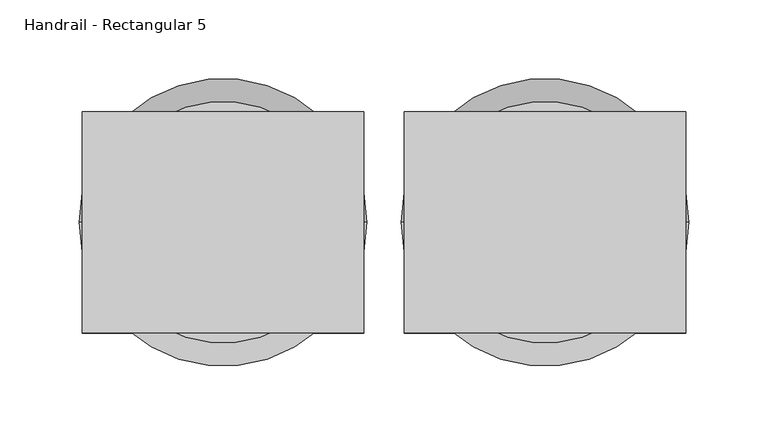
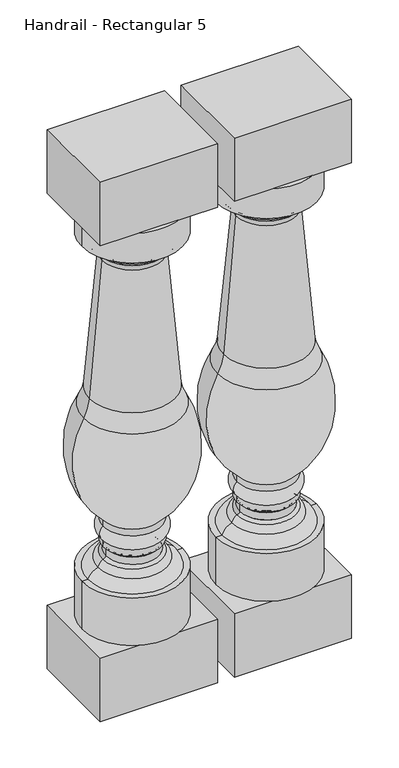
"""IFC4 building model written with IfcOpenShell, lengths in millimetres: railing geometry, Handrail - Rectangular 5."""

from ifc_helpers import new_model, si_unit, point, frame, origin, place, context, project, spatial, polyline, circle_curve, ellipse_curve, trimmed, outline, extrude, source, transform, mapped, element, save
from ifc_brep_helpers import plane_surface, cylinder_surface, revolved_surface, advanced_brep


def handrail_rectangular_5_6e42911b(model_context):
    return source(origin(), model_context, "Body", "SolidModel", [
        advanced_brep(
        [(16494.6521895, -1665.6164768, 873.125), (16647.0521895, -1665.6164768, 873.125), (16570.8521895, -1665.6164768, 873.125), (16494.6521895, -1665.6164768, 825.4490755), (16647.0521895, -1665.6164768, 825.4490755), (16504.6954208, -1665.6164768, 825.4490755), (16637.0089583, -1665.6164768, 825.4490755), (16516.1787107, -1665.6164768, 813.9657856), (16625.5256684, -1665.6164768, 813.9657856), (16516.1787107, -1665.6164768, 808.3461292), (16625.5256684, -1665.6164768, 808.3461292), (16521.8808978, -1665.6164768, 802.2016975), (16619.8234813, -1665.6164768, 802.2016975), (16525.2226936, -1665.6164768, 792.8428746), (16616.4816855, -1665.6164768, 792.8428746), (16506.4551876, -1665.6164768, 577.4758218), (16635.2491915, -1665.6164768, 577.4758218), (16497.437965, -1665.6164768, 549.5125844), (16644.2664141, -1665.6164768, 549.5125844), (16526.7087972, -1665.6164768, 376.7693301), (16614.9955818, -1665.6164768, 376.7693301), (16526.7087972, -1665.6164768, 366.4437154), (16614.9955818, -1665.6164768, 366.4437154), (16526.7087972, -1665.6164768, 343.8682651), (16614.9955818, -1665.6164768, 343.8682651), (16526.7087972, -1665.6164768, 333.5426504), (16614.9955818, -1665.6164768, 333.5426504), (16531.0192375, -1665.6164768, 329.2322102), (16610.6851416, -1665.6164768, 329.2322102), (16531.0192375, -1665.6164768, 317.4353211), (16610.6851416, -1665.6164768, 317.4353211), (16526.5214444, -1665.6164768, 313.1289544), (16615.1829347, -1665.6164768, 313.1289544), (16519.0009874, -1665.6164768, 303.0807869), (16622.7033917, -1665.6164768, 303.0807869), (16503.8523786, -1665.6164768, 288.925), (16637.8520004, -1665.6164768, 288.925), (16494.6521895, -1665.6164768, 288.925), (16647.0521895, -1665.6164768, 288.925), (16494.6521895, -1665.6164768, 212.725), (16647.0521895, -1665.6164768, 212.725), (16570.8521895, -1665.6164768, 212.725)],
        [
            (0, 1, circle_curve(frame((16570.8521895, -1665.6164768, 873.125), z_axis=(0.0, 0.0, 1.0), x_axis=(1.0, 0.0, 0.0)), 76.2)),
            (1, 2),
            (2, 0),
            (1, 0, circle_curve(frame((16570.8521895, -1665.6164768, 873.125), z_axis=(0.0, 0.0, 1.0), x_axis=(1.0, 0.0, 0.0)), 76.2)),
            (3, 4, circle_curve(frame((16570.8521895, -1665.6164768, 825.4490755), z_axis=(0.0, 0.0, 1.0), x_axis=(1.0, 0.0, 0.0)), 76.2)),
            (4, 1),
            (0, 3),
            (4, 3, circle_curve(frame((16570.8521895, -1665.6164768, 825.4490755), z_axis=(0.0, 0.0, 1.0), x_axis=(1.0, 0.0, 0.0)), 76.2)),
            (5, 6, circle_curve(frame((16570.8521895, -1665.6164768, 825.4490755), z_axis=(0.0, 0.0, 1.0), x_axis=(1.0, 0.0, 0.0)), 66.1567687)),
            (6, 4),
            (3, 5),
            (6, 5, circle_curve(frame((16570.8521895, -1665.6164768, 825.4490755), z_axis=(0.0, 0.0, 1.0), x_axis=(1.0, 0.0, 0.0)), 66.1567687)),
            (7, 8, circle_curve(frame((16570.8521895, -1665.6164768, 813.9657856), z_axis=(0.0, 0.0, 1.0), x_axis=(1.0, 0.0, 0.0)), 54.6734788)),
            (8, 6, circle_curve(frame((16625.5256684, -1665.6164768, 825.4490755), z_axis=(0.0, -1.0, 0.0), x_axis=(-1.0, 0.0, 0.0)), 11.4832899)),
            (5, 7, circle_curve(frame((16516.1787107, -1665.6164768, 825.4490755), z_axis=(0.0, -1.0, 0.0), x_axis=(1.0, 0.0, 0.0)), 11.4832899)),
            (8, 7, circle_curve(frame((16570.8521895, -1665.6164768, 813.9657856), z_axis=(0.0, 0.0, 1.0), x_axis=(1.0, 0.0, 0.0)), 54.6734788)),
            (9, 10, circle_curve(frame((16570.8521895, -1665.6164768, 808.3461292), z_axis=(0.0, 0.0, 1.0), x_axis=(1.0, 0.0, 0.0)), 54.6734788)),
            (10, 8),
            (7, 9),
            (10, 9, circle_curve(frame((16570.8521895, -1665.6164768, 808.3461292), z_axis=(0.0, 0.0, 1.0), x_axis=(1.0, 0.0, 0.0)), 54.6734788)),
            (11, 12, circle_curve(frame((16570.8521895, -1665.6164768, 802.2016975), z_axis=(0.0, 0.0, 1.0), x_axis=(1.0, 0.0, 0.0)), 48.9712918)),
            (12, 10, circle_curve(frame((16633.2345288, -1665.6164768, 795.4740105), z_axis=(0.0, 1.0, 0.0), x_axis=(-1.0, 0.0, 0.0)), 15.0039317)),
            (9, 11, circle_curve(frame((16508.4698503, -1665.6164768, 795.4740105), z_axis=(0.0, 1.0, 0.0), x_axis=(1.0, 0.0, 0.0)), 15.0039317)),
            (12, 11, circle_curve(frame((16570.8521895, -1665.6164768, 802.2016975), z_axis=(0.0, 0.0, 1.0), x_axis=(1.0, 0.0, 0.0)), 48.9712918)),
            (13, 14, circle_curve(frame((16570.8521895, -1665.6164768, 792.8428746), z_axis=(0.0, 0.0, 1.0), x_axis=(1.0, 0.0, 0.0)), 45.629496)),
            (14, 12, circle_curve(frame((16629.1595739, -1665.6164768, 793.5919719), z_axis=(0.0, 1.0, 0.0), x_axis=(-1.0, 0.0, 0.0)), 12.7)),
            (11, 13, circle_curve(frame((16512.5448052, -1665.6164768, 793.5919719), z_axis=(0.0, 1.0, 0.0), x_axis=(1.0, 0.0, 0.0)), 12.7)),
            (14, 13, circle_curve(frame((16570.8521895, -1665.6164768, 792.8428746), z_axis=(0.0, 0.0, 1.0), x_axis=(1.0, 0.0, 0.0)), 45.629496)),
            (15, 16, circle_curve(frame((16570.8521895, -1665.6164768, 577.4758218), z_axis=(0.0, 0.0, 1.0), x_axis=(1.0, 0.0, 0.0)), 64.3970019)),
            (16, 14, circle_curve(frame((20483.9232099, -1665.6164768, 1021.358044), z_axis=(0.0, 1.0, 0.0), x_axis=(-1.0, 0.0, 0.0)), 3874.1867698)),
            (13, 15, circle_curve(frame((12657.7811691, -1665.6164768, 1021.358044), z_axis=(0.0, 1.0, 0.0), x_axis=(1.0, 0.0, 0.0)), 3874.1867698)),
            (16, 15, circle_curve(frame((16570.8521895, -1665.6164768, 577.4758218), z_axis=(0.0, 0.0, 1.0), x_axis=(1.0, 0.0, 0.0)), 64.3970019)),
            (17, 18, circle_curve(frame((16570.8521895, -1665.6164768, 549.5125844), z_axis=(0.0, 0.0, 1.0), x_axis=(1.0, 0.0, 0.0)), 73.4142246)),
            (18, 16, circle_curve(frame((16709.7688441, -1665.6164768, 586.070457), z_axis=(0.0, 1.0, 0.0), x_axis=(-1.0, 0.0, 0.0)), 75.0136413)),
            (15, 17, circle_curve(frame((16431.935535, -1665.6164768, 586.070457), z_axis=(0.0, 1.0, 0.0), x_axis=(1.0, 0.0, 0.0)), 75.0136413)),
            (18, 17, circle_curve(frame((16570.8521895, -1665.6164768, 549.5125844), z_axis=(0.0, 0.0, 1.0), x_axis=(1.0, 0.0, 0.0)), 73.4142246)),
            (19, 20, circle_curve(frame((16570.8521895, -1665.6164768, 376.7693301), z_axis=(0.0, 0.0, 1.0), x_axis=(1.0, 0.0, 0.0)), 44.1433923)),
            (20, 18, circle_curve(frame((16522.1440648, -1665.6164768, 481.3542994), z_axis=(0.0, -1.0, 0.0), x_axis=(-1.0, 0.0, 0.0)), 139.8549964)),
            (17, 19, circle_curve(frame((16619.5603143, -1665.6164768, 481.3542994), z_axis=(0.0, -1.0, 0.0), x_axis=(1.0, 0.0, 0.0)), 139.8549964)),
            (20, 19, circle_curve(frame((16570.8521895, -1665.6164768, 376.7693301), z_axis=(0.0, 0.0, 1.0), x_axis=(1.0, 0.0, 0.0)), 44.1433923)),
            (21, 22, circle_curve(frame((16570.8521895, -1665.6164768, 366.4437154), z_axis=(0.0, 0.0, 1.0), x_axis=(1.0, 0.0, 0.0)), 44.1433923)),
            (22, 20),
            (19, 21),
            (22, 21, circle_curve(frame((16570.8521895, -1665.6164768, 366.4437154), z_axis=(0.0, 0.0, 1.0), x_axis=(1.0, 0.0, 0.0)), 44.1433923)),
            (23, 24, circle_curve(frame((16570.8521895, -1665.6164768, 343.8682651), z_axis=(0.0, 0.0, 1.0), x_axis=(1.0, 0.0, 0.0)), 44.1433923)),
            (24, 22, circle_curve(frame((16606.703554, -1665.6164768, 355.1559903), z_axis=(0.0, -1.0, 0.0), x_axis=(-1.0, 0.0, 0.0)), 14.0060867)),
            (21, 23, circle_curve(frame((16535.0008251, -1665.6164768, 355.1559903), z_axis=(0.0, -1.0, 0.0), x_axis=(1.0, 0.0, 0.0)), 14.0060867)),
            (24, 23, circle_curve(frame((16570.8521895, -1665.6164768, 343.8682651), z_axis=(0.0, 0.0, 1.0), x_axis=(1.0, 0.0, 0.0)), 44.1433923)),
            (25, 26, circle_curve(frame((16570.8521895, -1665.6164768, 333.5426504), z_axis=(0.0, 0.0, 1.0), x_axis=(1.0, 0.0, 0.0)), 44.1433923)),
            (26, 24),
            (23, 25),
            (26, 25, circle_curve(frame((16570.8521895, -1665.6164768, 333.5426504), z_axis=(0.0, 0.0, 1.0), x_axis=(1.0, 0.0, 0.0)), 44.1433923)),
            (27, 28, circle_curve(frame((16570.8521895, -1665.6164768, 329.2322102), z_axis=(0.0, 0.0, 1.0), x_axis=(1.0, 0.0, 0.0)), 39.8329521)),
            (28, 26, circle_curve(frame((16614.9955818, -1665.6164768, 329.2322102), z_axis=(0.0, 1.0, 0.0), x_axis=(-1.0, 0.0, 0.0)), 4.3104402)),
            (25, 27, circle_curve(frame((16526.7087972, -1665.6164768, 329.2322102), z_axis=(0.0, 1.0, 0.0), x_axis=(1.0, 0.0, 0.0)), 4.3104402)),
            (28, 27, circle_curve(frame((16570.8521895, -1665.6164768, 329.2322102), z_axis=(0.0, 0.0, 1.0), x_axis=(1.0, 0.0, 0.0)), 39.8329521)),
            (29, 30, circle_curve(frame((16570.8521895, -1665.6164768, 317.4353211), z_axis=(0.0, 0.0, 1.0), x_axis=(1.0, 0.0, 0.0)), 39.8329521)),
            (30, 28),
            (27, 29),
            (30, 29, circle_curve(frame((16570.8521895, -1665.6164768, 317.4353211), z_axis=(0.0, 0.0, 1.0), x_axis=(1.0, 0.0, 0.0)), 39.8329521)),
            (31, 32, circle_curve(frame((16570.8521895, -1665.6164768, 313.1289544), z_axis=(0.0, 0.0, 1.0), x_axis=(1.0, 0.0, 0.0)), 44.3307451)),
            (32, 30, circle_curve(frame((16614.9955818, -1665.6164768, 317.4353211), z_axis=(0.0, 1.0, 0.0), x_axis=(-1.0, 0.0, 0.0)), 4.3104402)),
            (29, 31, circle_curve(frame((16526.7087972, -1665.6164768, 317.4353211), z_axis=(0.0, 1.0, 0.0), x_axis=(1.0, 0.0, 0.0)), 4.3104402)),
            (32, 31, circle_curve(frame((16570.8521895, -1665.6164768, 313.1289544), z_axis=(0.0, 0.0, 1.0), x_axis=(1.0, 0.0, 0.0)), 44.3307451)),
            (33, 34, circle_curve(frame((16570.8521895, -1665.6164768, 303.0807869), z_axis=(0.0, 0.0, 1.0), x_axis=(1.0, 0.0, 0.0)), 51.8512022)),
            (34, 32, circle_curve(frame((16608.0640754, -1665.6164768, 299.962519), z_axis=(0.0, -1.0, 0.0), x_axis=(-1.0, 0.0, 0.0)), 14.9677378)),
            (31, 33, circle_curve(frame((16533.6403037, -1665.6164768, 299.962519), z_axis=(0.0, -1.0, 0.0), x_axis=(1.0, 0.0, 0.0)), 14.9677378)),
            (34, 33, circle_curve(frame((16570.8521895, -1665.6164768, 303.0807869), z_axis=(0.0, 0.0, 1.0), x_axis=(1.0, 0.0, 0.0)), 51.8512022)),
            (35, 36, circle_curve(frame((16570.8521895, -1665.6164768, 288.925), z_axis=(0.0, 0.0, 1.0), x_axis=(1.0, 0.0, 0.0)), 66.9998109)),
            (36, 34, circle_curve(frame((16617.4545436, -1665.6164768, 282.2803841), z_axis=(0.0, -1.0, 0.0), x_axis=(-1.0, 0.0, 0.0)), 21.4524396)),
            (33, 35, circle_curve(frame((16524.2498354, -1665.6164768, 282.2803841), z_axis=(0.0, -1.0, 0.0), x_axis=(1.0, 0.0, 0.0)), 21.4524396)),
            (36, 35, circle_curve(frame((16570.8521895, -1665.6164768, 288.925), z_axis=(0.0, 0.0, 1.0), x_axis=(1.0, 0.0, 0.0)), 66.9998109)),
            (37, 38, circle_curve(frame((16570.8521895, -1665.6164768, 288.925), z_axis=(0.0, 0.0, 1.0), x_axis=(1.0, 0.0, 0.0)), 76.2)),
            (38, 36),
            (35, 37),
            (38, 37, circle_curve(frame((16570.8521895, -1665.6164768, 288.925), z_axis=(0.0, 0.0, 1.0), x_axis=(1.0, 0.0, 0.0)), 76.2)),
            (39, 40, circle_curve(frame((16570.8521895, -1665.6164768, 212.725), z_axis=(0.0, 0.0, 1.0), x_axis=(1.0, 0.0, 0.0)), 76.2)),
            (40, 38),
            (37, 39),
            (40, 39, circle_curve(frame((16570.8521895, -1665.6164768, 212.725), z_axis=(0.0, 0.0, 1.0), x_axis=(1.0, 0.0, 0.0)), 76.2)),
            (41, 40),
            (39, 41),
        ],
        [
            plane_surface(frame((16570.8521895, -1665.6164768, 873.125), z_axis=(0.0, 0.0, 1.0), x_axis=(1.0, 0.0, 0.0))),
            cylinder_surface(frame((16570.8521895, -1665.6164768, 841.375), z_axis=(0.0, 0.0, -1.0), x_axis=(1.0, 0.0, 0.0)), 76.2),
            plane_surface(frame((16570.8521895, -1665.6164768, 825.4490755), z_axis=(0.0, 0.0, -1.0), x_axis=(1.0, 0.0, 0.0))),
            revolved_surface(trimmed(ellipse_curve(frame((16625.5256684, -1665.6164768, 825.4490755), z_axis=(0.0, 1.0, 0.0), x_axis=(-1.0, 0.0, 0.0)), 11.4832899, 11.4832899), [point((16637.0089583, -1665.6164768, 825.4490755))], [point((16625.5256684, -1665.6164768, 813.9657856))], True, "CARTESIAN"), (16570.8521895, -1665.6164768, 841.375), (0.0, 0.0, -1.0)),
            cylinder_surface(frame((16570.8521895, -1665.6164768, 841.375), z_axis=(0.0, 0.0, -1.0), x_axis=(1.0, 0.0, 0.0)), 54.6734788),
            revolved_surface(trimmed(ellipse_curve(frame((16633.2345288, -1665.6164768, 795.4740105), z_axis=(0.0, -1.0, 0.0), x_axis=(-1.0, 0.0, 0.0)), 15.0039317, 15.0039317), [point((16625.5256684, -1665.6164768, 808.3461292))], [point((16619.8234813, -1665.6164768, 802.2016975))], True, "CARTESIAN"), (16570.8521895, -1665.6164768, 841.375), (0.0, 0.0, -1.0)),
            revolved_surface(trimmed(ellipse_curve(frame((16629.1595739, -1665.6164768, 793.5919719), z_axis=(0.0, -1.0, 0.0), x_axis=(-1.0, 0.0, 0.0)), 12.7, 12.7), [point((16619.8234813, -1665.6164768, 802.2016975))], [point((16616.4816855, -1665.6164768, 792.8428746))], True, "CARTESIAN"), (16570.8521895, -1665.6164768, 841.375), (0.0, 0.0, -1.0)),
            revolved_surface(trimmed(ellipse_curve(frame((20483.9232099, -1665.6164768, 1021.358044), z_axis=(0.0, -1.0, 0.0), x_axis=(-1.0, 0.0, 0.0)), 3874.1867698, 3874.1867698), [point((16616.4816855, -1665.6164768, 792.8428746))], [point((16635.2491915, -1665.6164768, 577.4758218))], True, "CARTESIAN"), (16570.8521895, -1665.6164768, 841.375), (0.0, 0.0, -1.0)),
            revolved_surface(trimmed(ellipse_curve(frame((16709.7688441, -1665.6164768, 586.070457), z_axis=(0.0, -1.0, 0.0), x_axis=(-1.0, 0.0, 0.0)), 75.0136413, 75.0136413), [point((16635.2491915, -1665.6164768, 577.4758218))], [point((16644.2664141, -1665.6164768, 549.5125844))], True, "CARTESIAN"), (16570.8521895, -1665.6164768, 841.375), (0.0, 0.0, -1.0)),
            revolved_surface(trimmed(ellipse_curve(frame((16522.1440648, -1665.6164768, 481.3542994), z_axis=(0.0, 1.0, 0.0), x_axis=(-1.0, 0.0, 0.0)), 139.8549964, 139.8549964), [point((16644.2664141, -1665.6164768, 549.5125844))], [point((16614.9955818, -1665.6164768, 376.7693301))], True, "CARTESIAN"), (16570.8521895, -1665.6164768, 841.375), (0.0, 0.0, -1.0)),
            cylinder_surface(frame((16570.8521895, -1665.6164768, 841.375), z_axis=(0.0, 0.0, -1.0), x_axis=(1.0, 0.0, 0.0)), 44.1433923),
            revolved_surface(trimmed(ellipse_curve(frame((16606.703554, -1665.6164768, 355.1559903), z_axis=(0.0, 1.0, 0.0), x_axis=(-1.0, 0.0, 0.0)), 14.0060867, 14.0060867), [point((16614.9955818, -1665.6164768, 366.4437154))], [point((16614.9955818, -1665.6164768, 343.8682651))], True, "CARTESIAN"), (16570.8521895, -1665.6164768, 841.375), (0.0, 0.0, -1.0)),
            revolved_surface(trimmed(ellipse_curve(frame((16614.9955818, -1665.6164768, 329.2322102), z_axis=(0.0, -1.0, 0.0), x_axis=(-1.0, 0.0, 0.0)), 4.3104402, 4.3104402), [point((16614.9955818, -1665.6164768, 333.5426504))], [point((16610.6851416, -1665.6164768, 329.2322102))], True, "CARTESIAN"), (16570.8521895, -1665.6164768, 841.375), (0.0, 0.0, -1.0)),
            cylinder_surface(frame((16570.8521895, -1665.6164768, 841.375), z_axis=(0.0, 0.0, -1.0), x_axis=(1.0, 0.0, 0.0)), 39.8329521),
            revolved_surface(trimmed(ellipse_curve(frame((16614.9955818, -1665.6164768, 317.4353211), z_axis=(0.0, -1.0, 0.0), x_axis=(-1.0, 0.0, 0.0)), 4.3104402, 4.3104402), [point((16610.6851416, -1665.6164768, 317.4353211))], [point((16615.1829347, -1665.6164768, 313.1289544))], True, "CARTESIAN"), (16570.8521895, -1665.6164768, 841.375), (0.0, 0.0, -1.0)),
            revolved_surface(trimmed(ellipse_curve(frame((16608.0640754, -1665.6164768, 299.962519), z_axis=(0.0, 1.0, 0.0), x_axis=(-1.0, 0.0, 0.0)), 14.9677378, 14.9677378), [point((16615.1829347, -1665.6164768, 313.1289544))], [point((16622.7033917, -1665.6164768, 303.0807869))], True, "CARTESIAN"), (16570.8521895, -1665.6164768, 841.375), (0.0, 0.0, -1.0)),
            revolved_surface(trimmed(ellipse_curve(frame((16617.4545436, -1665.6164768, 282.2803841), z_axis=(0.0, 1.0, 0.0), x_axis=(-1.0, 0.0, 0.0)), 21.4524396, 21.4524396), [point((16622.7033917, -1665.6164768, 303.0807869))], [point((16637.8520004, -1665.6164768, 288.925))], True, "CARTESIAN"), (16570.8521895, -1665.6164768, 841.375), (0.0, 0.0, -1.0)),
            plane_surface(frame((16570.8521895, -1665.6164768, 288.925), z_axis=(0.0, 0.0, 1.0), x_axis=(1.0, 0.0, 0.0))),
            plane_surface(frame((16570.8521895, -1665.6164768, 212.725), z_axis=(0.0, 0.0, -1.0), x_axis=(1.0, 0.0, 0.0))),
        ],
        [
            (0, [[1, 2, 3]]),
            (0, [[4, -3, -2]]),
            (1, [[5, 6, -1, 7]]),
            (1, [[8, -7, -4, -6]]),
            (2, [[9, 10, -5, 11]]),
            (2, [[12, -11, -8, -10]]),
            (3, [[13, 14, -9, 15]]),
            (3, [[16, -15, -12, -14]]),
            (4, [[17, 18, -13, 19]]),
            (4, [[20, -19, -16, -18]]),
            (5, [[21, 22, -17, 23]]),
            (5, [[24, -23, -20, -22]]),
            (6, [[25, 26, -21, 27]]),
            (6, [[28, -27, -24, -26]]),
            (7, [[29, 30, -25, 31]]),
            (7, [[32, -31, -28, -30]]),
            (8, [[33, 34, -29, 35]]),
            (8, [[36, -35, -32, -34]]),
            (9, [[37, 38, -33, 39]]),
            (9, [[40, -39, -36, -38]]),
            (10, [[41, 42, -37, 43]]),
            (10, [[44, -43, -40, -42]]),
            (11, [[45, 46, -41, 47]]),
            (11, [[48, -47, -44, -46]]),
            (10, [[49, 50, -45, 51]]),
            (10, [[52, -51, -48, -50]]),
            (12, [[53, 54, -49, 55]]),
            (12, [[56, -55, -52, -54]]),
            (13, [[57, 58, -53, 59]]),
            (13, [[60, -59, -56, -58]]),
            (14, [[61, 62, -57, 63]]),
            (14, [[64, -63, -60, -62]]),
            (15, [[65, 66, -61, 67]]),
            (15, [[68, -67, -64, -66]]),
            (16, [[69, 70, -65, 71]]),
            (16, [[72, -71, -68, -70]]),
            (17, [[73, 74, -69, 75]]),
            (17, [[76, -75, -72, -74]]),
            (1, [[77, 78, -73, 79]]),
            (1, [[80, -79, -76, -78]]),
            (18, [[81, -77, 82]]),
            (18, [[-82, -80, -81]]),
        ],
    ),
        extrude(outline(polyline([(16481.9521895, -1735.4664768), (16481.9521895, -1595.7664768), (16659.7521895, -1595.7664768), (16659.7521895, -1735.4664768), (16481.9521895, -1735.4664768)])), frame((0.0, 0.0, 111.125), z_axis=(0.0, 0.0, 1.0), x_axis=(1.0, 0.0, 0.0)), (0.0, 0.0, 1.0), 101.6),
        extrude(outline(polyline([(16481.9521895, -1595.7664768), (16659.7521895, -1595.7664768), (16659.7521895, -1735.4664768), (16481.9521895, -1735.4664768), (16481.9521895, -1595.7664768)])), frame((0.0, 0.0, 873.125), z_axis=(0.0, 0.0, 1.0), x_axis=(1.0, 0.0, 0.0)), (0.0, 0.0, 1.0), 101.6),
        advanced_brep(
        [(16291.4521895, -1665.6164768, 873.125), (16443.8521895, -1665.6164768, 873.125), (16367.6521895, -1665.6164768, 873.125), (16291.4521895, -1665.6164768, 825.4490755), (16443.8521895, -1665.6164768, 825.4490755), (16301.4954208, -1665.6164768, 825.4490755), (16433.8089583, -1665.6164768, 825.4490755), (16312.9787107, -1665.6164768, 813.9657856), (16422.3256684, -1665.6164768, 813.9657856), (16312.9787107, -1665.6164768, 808.3461292), (16422.3256684, -1665.6164768, 808.3461292), (16318.6808978, -1665.6164768, 802.2016975), (16416.6234813, -1665.6164768, 802.2016975), (16322.0226936, -1665.6164768, 792.8428746), (16413.2816855, -1665.6164768, 792.8428746), (16303.2551876, -1665.6164768, 577.4758218), (16432.0491915, -1665.6164768, 577.4758218), (16294.237965, -1665.6164768, 549.5125844), (16441.0664141, -1665.6164768, 549.5125844), (16323.5087972, -1665.6164768, 376.7693301), (16411.7955818, -1665.6164768, 376.7693301), (16323.5087972, -1665.6164768, 366.4437154), (16411.7955818, -1665.6164768, 366.4437154), (16323.5087972, -1665.6164768, 343.8682651), (16411.7955818, -1665.6164768, 343.8682651), (16323.5087972, -1665.6164768, 333.5426504), (16411.7955818, -1665.6164768, 333.5426504), (16327.8192375, -1665.6164768, 329.2322102), (16407.4851416, -1665.6164768, 329.2322102), (16327.8192375, -1665.6164768, 317.4353211), (16407.4851416, -1665.6164768, 317.4353211), (16323.3214444, -1665.6164768, 313.1289544), (16411.9829347, -1665.6164768, 313.1289544), (16315.8009874, -1665.6164768, 303.0807869), (16419.5033917, -1665.6164768, 303.0807869), (16300.6523786, -1665.6164768, 288.925), (16434.6520004, -1665.6164768, 288.925), (16291.4521895, -1665.6164768, 288.925), (16443.8521895, -1665.6164768, 288.925), (16291.4521895, -1665.6164768, 212.725), (16443.8521895, -1665.6164768, 212.725), (16367.6521895, -1665.6164768, 212.725)],
        [
            (0, 1, circle_curve(frame((16367.6521895, -1665.6164768, 873.125), z_axis=(0.0, 0.0, 1.0), x_axis=(1.0, 0.0, 0.0)), 76.2)),
            (1, 2),
            (2, 0),
            (1, 0, circle_curve(frame((16367.6521895, -1665.6164768, 873.125), z_axis=(0.0, 0.0, 1.0), x_axis=(1.0, 0.0, 0.0)), 76.2)),
            (3, 4, circle_curve(frame((16367.6521895, -1665.6164768, 825.4490755), z_axis=(0.0, 0.0, 1.0), x_axis=(1.0, 0.0, 0.0)), 76.2)),
            (4, 1),
            (0, 3),
            (4, 3, circle_curve(frame((16367.6521895, -1665.6164768, 825.4490755), z_axis=(0.0, 0.0, 1.0), x_axis=(1.0, 0.0, 0.0)), 76.2)),
            (5, 6, circle_curve(frame((16367.6521895, -1665.6164768, 825.4490755), z_axis=(0.0, 0.0, 1.0), x_axis=(1.0, 0.0, 0.0)), 66.1567687)),
            (6, 4),
            (3, 5),
            (6, 5, circle_curve(frame((16367.6521895, -1665.6164768, 825.4490755), z_axis=(0.0, 0.0, 1.0), x_axis=(1.0, 0.0, 0.0)), 66.1567687)),
            (7, 8, circle_curve(frame((16367.6521895, -1665.6164768, 813.9657856), z_axis=(0.0, 0.0, 1.0), x_axis=(1.0, 0.0, 0.0)), 54.6734788)),
            (8, 6, circle_curve(frame((16422.3256684, -1665.6164768, 825.4490755), z_axis=(0.0, -1.0, 0.0), x_axis=(-1.0, 0.0, 0.0)), 11.4832899)),
            (5, 7, circle_curve(frame((16312.9787107, -1665.6164768, 825.4490755), z_axis=(0.0, -1.0, 0.0), x_axis=(1.0, 0.0, 0.0)), 11.4832899)),
            (8, 7, circle_curve(frame((16367.6521895, -1665.6164768, 813.9657856), z_axis=(0.0, 0.0, 1.0), x_axis=(1.0, 0.0, 0.0)), 54.6734788)),
            (9, 10, circle_curve(frame((16367.6521895, -1665.6164768, 808.3461292), z_axis=(0.0, 0.0, 1.0), x_axis=(1.0, 0.0, 0.0)), 54.6734788)),
            (10, 8),
            (7, 9),
            (10, 9, circle_curve(frame((16367.6521895, -1665.6164768, 808.3461292), z_axis=(0.0, 0.0, 1.0), x_axis=(1.0, 0.0, 0.0)), 54.6734788)),
            (11, 12, circle_curve(frame((16367.6521895, -1665.6164768, 802.2016975), z_axis=(0.0, 0.0, 1.0), x_axis=(1.0, 0.0, 0.0)), 48.9712918)),
            (12, 10, circle_curve(frame((16430.0345288, -1665.6164768, 795.4740105), z_axis=(0.0, 1.0, 0.0), x_axis=(-1.0, 0.0, 0.0)), 15.0039317)),
            (9, 11, circle_curve(frame((16305.2698503, -1665.6164768, 795.4740105), z_axis=(0.0, 1.0, 0.0), x_axis=(1.0, 0.0, 0.0)), 15.0039317)),
            (12, 11, circle_curve(frame((16367.6521895, -1665.6164768, 802.2016975), z_axis=(0.0, 0.0, 1.0), x_axis=(1.0, 0.0, 0.0)), 48.9712918)),
            (13, 14, circle_curve(frame((16367.6521895, -1665.6164768, 792.8428746), z_axis=(0.0, 0.0, 1.0), x_axis=(1.0, 0.0, 0.0)), 45.629496)),
            (14, 12, circle_curve(frame((16425.9595739, -1665.6164768, 793.5919719), z_axis=(0.0, 1.0, 0.0), x_axis=(-1.0, 0.0, 0.0)), 12.7)),
            (11, 13, circle_curve(frame((16309.3448052, -1665.6164768, 793.5919719), z_axis=(0.0, 1.0, 0.0), x_axis=(1.0, 0.0, 0.0)), 12.7)),
            (14, 13, circle_curve(frame((16367.6521895, -1665.6164768, 792.8428746), z_axis=(0.0, 0.0, 1.0), x_axis=(1.0, 0.0, 0.0)), 45.629496)),
            (15, 16, circle_curve(frame((16367.6521895, -1665.6164768, 577.4758218), z_axis=(0.0, 0.0, 1.0), x_axis=(1.0, 0.0, 0.0)), 64.3970019)),
            (16, 14, circle_curve(frame((20280.7232099, -1665.6164768, 1021.358044), z_axis=(0.0, 1.0, 0.0), x_axis=(-1.0, 0.0, 0.0)), 3874.1867698)),
            (13, 15, circle_curve(frame((12454.5811691, -1665.6164768, 1021.358044), z_axis=(0.0, 1.0, 0.0), x_axis=(1.0, 0.0, 0.0)), 3874.1867698)),
            (16, 15, circle_curve(frame((16367.6521895, -1665.6164768, 577.4758218), z_axis=(0.0, 0.0, 1.0), x_axis=(1.0, 0.0, 0.0)), 64.3970019)),
            (17, 18, circle_curve(frame((16367.6521895, -1665.6164768, 549.5125844), z_axis=(0.0, 0.0, 1.0), x_axis=(1.0, 0.0, 0.0)), 73.4142246)),
            (18, 16, circle_curve(frame((16506.5688441, -1665.6164768, 586.070457), z_axis=(0.0, 1.0, 0.0), x_axis=(-1.0, 0.0, 0.0)), 75.0136413)),
            (15, 17, circle_curve(frame((16228.735535, -1665.6164768, 586.070457), z_axis=(0.0, 1.0, 0.0), x_axis=(1.0, 0.0, 0.0)), 75.0136413)),
            (18, 17, circle_curve(frame((16367.6521895, -1665.6164768, 549.5125844), z_axis=(0.0, 0.0, 1.0), x_axis=(1.0, 0.0, 0.0)), 73.4142246)),
            (19, 20, circle_curve(frame((16367.6521895, -1665.6164768, 376.7693301), z_axis=(0.0, 0.0, 1.0), x_axis=(1.0, 0.0, 0.0)), 44.1433923)),
            (20, 18, circle_curve(frame((16318.9440648, -1665.6164768, 481.3542994), z_axis=(0.0, -1.0, 0.0), x_axis=(-1.0, 0.0, 0.0)), 139.8549964)),
            (17, 19, circle_curve(frame((16416.3603143, -1665.6164768, 481.3542994), z_axis=(0.0, -1.0, 0.0), x_axis=(1.0, 0.0, 0.0)), 139.8549964)),
            (20, 19, circle_curve(frame((16367.6521895, -1665.6164768, 376.7693301), z_axis=(0.0, 0.0, 1.0), x_axis=(1.0, 0.0, 0.0)), 44.1433923)),
            (21, 22, circle_curve(frame((16367.6521895, -1665.6164768, 366.4437154), z_axis=(0.0, 0.0, 1.0), x_axis=(1.0, 0.0, 0.0)), 44.1433923)),
            (22, 20),
            (19, 21),
            (22, 21, circle_curve(frame((16367.6521895, -1665.6164768, 366.4437154), z_axis=(0.0, 0.0, 1.0), x_axis=(1.0, 0.0, 0.0)), 44.1433923)),
            (23, 24, circle_curve(frame((16367.6521895, -1665.6164768, 343.8682651), z_axis=(0.0, 0.0, 1.0), x_axis=(1.0, 0.0, 0.0)), 44.1433923)),
            (24, 22, circle_curve(frame((16403.503554, -1665.6164768, 355.1559903), z_axis=(0.0, -1.0, 0.0), x_axis=(-1.0, 0.0, 0.0)), 14.0060867)),
            (21, 23, circle_curve(frame((16331.8008251, -1665.6164768, 355.1559903), z_axis=(0.0, -1.0, 0.0), x_axis=(1.0, 0.0, 0.0)), 14.0060867)),
            (24, 23, circle_curve(frame((16367.6521895, -1665.6164768, 343.8682651), z_axis=(0.0, 0.0, 1.0), x_axis=(1.0, 0.0, 0.0)), 44.1433923)),
            (25, 26, circle_curve(frame((16367.6521895, -1665.6164768, 333.5426504), z_axis=(0.0, 0.0, 1.0), x_axis=(1.0, 0.0, 0.0)), 44.1433923)),
            (26, 24),
            (23, 25),
            (26, 25, circle_curve(frame((16367.6521895, -1665.6164768, 333.5426504), z_axis=(0.0, 0.0, 1.0), x_axis=(1.0, 0.0, 0.0)), 44.1433923)),
            (27, 28, circle_curve(frame((16367.6521895, -1665.6164768, 329.2322102), z_axis=(0.0, 0.0, 1.0), x_axis=(1.0, 0.0, 0.0)), 39.8329521)),
            (28, 26, circle_curve(frame((16411.7955818, -1665.6164768, 329.2322102), z_axis=(0.0, 1.0, 0.0), x_axis=(-1.0, 0.0, 0.0)), 4.3104402)),
            (25, 27, circle_curve(frame((16323.5087972, -1665.6164768, 329.2322102), z_axis=(0.0, 1.0, 0.0), x_axis=(1.0, 0.0, 0.0)), 4.3104402)),
            (28, 27, circle_curve(frame((16367.6521895, -1665.6164768, 329.2322102), z_axis=(0.0, 0.0, 1.0), x_axis=(1.0, 0.0, 0.0)), 39.8329521)),
            (29, 30, circle_curve(frame((16367.6521895, -1665.6164768, 317.4353211), z_axis=(0.0, 0.0, 1.0), x_axis=(1.0, 0.0, 0.0)), 39.8329521)),
            (30, 28),
            (27, 29),
            (30, 29, circle_curve(frame((16367.6521895, -1665.6164768, 317.4353211), z_axis=(0.0, 0.0, 1.0), x_axis=(1.0, 0.0, 0.0)), 39.8329521)),
            (31, 32, circle_curve(frame((16367.6521895, -1665.6164768, 313.1289544), z_axis=(0.0, 0.0, 1.0), x_axis=(1.0, 0.0, 0.0)), 44.3307451)),
            (32, 30, circle_curve(frame((16411.7955818, -1665.6164768, 317.4353211), z_axis=(0.0, 1.0, 0.0), x_axis=(-1.0, 0.0, 0.0)), 4.3104402)),
            (29, 31, circle_curve(frame((16323.5087972, -1665.6164768, 317.4353211), z_axis=(0.0, 1.0, 0.0), x_axis=(1.0, 0.0, 0.0)), 4.3104402)),
            (32, 31, circle_curve(frame((16367.6521895, -1665.6164768, 313.1289544), z_axis=(0.0, 0.0, 1.0), x_axis=(1.0, 0.0, 0.0)), 44.3307451)),
            (33, 34, circle_curve(frame((16367.6521895, -1665.6164768, 303.0807869), z_axis=(0.0, 0.0, 1.0), x_axis=(1.0, 0.0, 0.0)), 51.8512022)),
            (34, 32, circle_curve(frame((16404.8640754, -1665.6164768, 299.962519), z_axis=(0.0, -1.0, 0.0), x_axis=(-1.0, 0.0, 0.0)), 14.9677378)),
            (31, 33, circle_curve(frame((16330.4403037, -1665.6164768, 299.962519), z_axis=(0.0, -1.0, 0.0), x_axis=(1.0, 0.0, 0.0)), 14.9677378)),
            (34, 33, circle_curve(frame((16367.6521895, -1665.6164768, 303.0807869), z_axis=(0.0, 0.0, 1.0), x_axis=(1.0, 0.0, 0.0)), 51.8512022)),
            (35, 36, circle_curve(frame((16367.6521895, -1665.6164768, 288.925), z_axis=(0.0, 0.0, 1.0), x_axis=(1.0, 0.0, 0.0)), 66.9998109)),
            (36, 34, circle_curve(frame((16414.2545436, -1665.6164768, 282.2803841), z_axis=(0.0, -1.0, 0.0), x_axis=(-1.0, 0.0, 0.0)), 21.4524396)),
            (33, 35, circle_curve(frame((16321.0498354, -1665.6164768, 282.2803841), z_axis=(0.0, -1.0, 0.0), x_axis=(1.0, 0.0, 0.0)), 21.4524396)),
            (36, 35, circle_curve(frame((16367.6521895, -1665.6164768, 288.925), z_axis=(0.0, 0.0, 1.0), x_axis=(1.0, 0.0, 0.0)), 66.9998109)),
            (37, 38, circle_curve(frame((16367.6521895, -1665.6164768, 288.925), z_axis=(0.0, 0.0, 1.0), x_axis=(1.0, 0.0, 0.0)), 76.2)),
            (38, 36),
            (35, 37),
            (38, 37, circle_curve(frame((16367.6521895, -1665.6164768, 288.925), z_axis=(0.0, 0.0, 1.0), x_axis=(1.0, 0.0, 0.0)), 76.2)),
            (39, 40, circle_curve(frame((16367.6521895, -1665.6164768, 212.725), z_axis=(0.0, 0.0, 1.0), x_axis=(1.0, 0.0, 0.0)), 76.2)),
            (40, 38),
            (37, 39),
            (40, 39, circle_curve(frame((16367.6521895, -1665.6164768, 212.725), z_axis=(0.0, 0.0, 1.0), x_axis=(1.0, 0.0, 0.0)), 76.2)),
            (41, 40),
            (39, 41),
        ],
        [
            plane_surface(frame((16367.6521895, -1665.6164768, 873.125), z_axis=(0.0, 0.0, 1.0), x_axis=(1.0, 0.0, 0.0))),
            cylinder_surface(frame((16367.6521895, -1665.6164768, 841.375), z_axis=(0.0, 0.0, -1.0), x_axis=(1.0, 0.0, 0.0)), 76.2),
            plane_surface(frame((16367.6521895, -1665.6164768, 825.4490755), z_axis=(0.0, 0.0, -1.0), x_axis=(1.0, 0.0, 0.0))),
            revolved_surface(trimmed(ellipse_curve(frame((16422.3256684, -1665.6164768, 825.4490755), z_axis=(0.0, 1.0, 0.0), x_axis=(-1.0, 0.0, 0.0)), 11.4832899, 11.4832899), [point((16433.8089583, -1665.6164768, 825.4490755))], [point((16422.3256684, -1665.6164768, 813.9657856))], True, "CARTESIAN"), (16367.6521895, -1665.6164768, 841.375), (0.0, 0.0, -1.0)),
            cylinder_surface(frame((16367.6521895, -1665.6164768, 841.375), z_axis=(0.0, 0.0, -1.0), x_axis=(1.0, 0.0, 0.0)), 54.6734788),
            revolved_surface(trimmed(ellipse_curve(frame((16430.0345288, -1665.6164768, 795.4740105), z_axis=(0.0, -1.0, 0.0), x_axis=(-1.0, 0.0, 0.0)), 15.0039317, 15.0039317), [point((16422.3256684, -1665.6164768, 808.3461292))], [point((16416.6234813, -1665.6164768, 802.2016975))], True, "CARTESIAN"), (16367.6521895, -1665.6164768, 841.375), (0.0, 0.0, -1.0)),
            revolved_surface(trimmed(ellipse_curve(frame((16425.9595739, -1665.6164768, 793.5919719), z_axis=(0.0, -1.0, 0.0), x_axis=(-1.0, 0.0, 0.0)), 12.7, 12.7), [point((16416.6234813, -1665.6164768, 802.2016975))], [point((16413.2816855, -1665.6164768, 792.8428746))], True, "CARTESIAN"), (16367.6521895, -1665.6164768, 841.375), (0.0, 0.0, -1.0)),
            revolved_surface(trimmed(ellipse_curve(frame((20280.7232099, -1665.6164768, 1021.358044), z_axis=(0.0, -1.0, 0.0), x_axis=(-1.0, 0.0, 0.0)), 3874.1867698, 3874.1867698), [point((16413.2816855, -1665.6164768, 792.8428746))], [point((16432.0491915, -1665.6164768, 577.4758218))], True, "CARTESIAN"), (16367.6521895, -1665.6164768, 841.375), (0.0, 0.0, -1.0)),
            revolved_surface(trimmed(ellipse_curve(frame((16506.5688441, -1665.6164768, 586.070457), z_axis=(0.0, -1.0, 0.0), x_axis=(-1.0, 0.0, 0.0)), 75.0136413, 75.0136413), [point((16432.0491915, -1665.6164768, 577.4758218))], [point((16441.0664141, -1665.6164768, 549.5125844))], True, "CARTESIAN"), (16367.6521895, -1665.6164768, 841.375), (0.0, 0.0, -1.0)),
            revolved_surface(trimmed(ellipse_curve(frame((16318.9440648, -1665.6164768, 481.3542994), z_axis=(0.0, 1.0, 0.0), x_axis=(-1.0, 0.0, 0.0)), 139.8549964, 139.8549964), [point((16441.0664141, -1665.6164768, 549.5125844))], [point((16411.7955818, -1665.6164768, 376.7693301))], True, "CARTESIAN"), (16367.6521895, -1665.6164768, 841.375), (0.0, 0.0, -1.0)),
            cylinder_surface(frame((16367.6521895, -1665.6164768, 841.375), z_axis=(0.0, 0.0, -1.0), x_axis=(1.0, 0.0, 0.0)), 44.1433923),
            revolved_surface(trimmed(ellipse_curve(frame((16403.503554, -1665.6164768, 355.1559903), z_axis=(0.0, 1.0, 0.0), x_axis=(-1.0, 0.0, 0.0)), 14.0060867, 14.0060867), [point((16411.7955818, -1665.6164768, 366.4437154))], [point((16411.7955818, -1665.6164768, 343.8682651))], True, "CARTESIAN"), (16367.6521895, -1665.6164768, 841.375), (0.0, 0.0, -1.0)),
            revolved_surface(trimmed(ellipse_curve(frame((16411.7955818, -1665.6164768, 329.2322102), z_axis=(0.0, -1.0, 0.0), x_axis=(-1.0, 0.0, 0.0)), 4.3104402, 4.3104402), [point((16411.7955818, -1665.6164768, 333.5426504))], [point((16407.4851416, -1665.6164768, 329.2322102))], True, "CARTESIAN"), (16367.6521895, -1665.6164768, 841.375), (0.0, 0.0, -1.0)),
            cylinder_surface(frame((16367.6521895, -1665.6164768, 841.375), z_axis=(0.0, 0.0, -1.0), x_axis=(1.0, 0.0, 0.0)), 39.8329521),
            revolved_surface(trimmed(ellipse_curve(frame((16411.7955818, -1665.6164768, 317.4353211), z_axis=(0.0, -1.0, 0.0), x_axis=(-1.0, 0.0, 0.0)), 4.3104402, 4.3104402), [point((16407.4851416, -1665.6164768, 317.4353211))], [point((16411.9829347, -1665.6164768, 313.1289544))], True, "CARTESIAN"), (16367.6521895, -1665.6164768, 841.375), (0.0, 0.0, -1.0)),
            revolved_surface(trimmed(ellipse_curve(frame((16404.8640754, -1665.6164768, 299.962519), z_axis=(0.0, 1.0, 0.0), x_axis=(-1.0, 0.0, 0.0)), 14.9677378, 14.9677378), [point((16411.9829347, -1665.6164768, 313.1289544))], [point((16419.5033917, -1665.6164768, 303.0807869))], True, "CARTESIAN"), (16367.6521895, -1665.6164768, 841.375), (0.0, 0.0, -1.0)),
            revolved_surface(trimmed(ellipse_curve(frame((16414.2545436, -1665.6164768, 282.2803841), z_axis=(0.0, 1.0, 0.0), x_axis=(-1.0, 0.0, 0.0)), 21.4524396, 21.4524396), [point((16419.5033917, -1665.6164768, 303.0807869))], [point((16434.6520004, -1665.6164768, 288.925))], True, "CARTESIAN"), (16367.6521895, -1665.6164768, 841.375), (0.0, 0.0, -1.0)),
            plane_surface(frame((16367.6521895, -1665.6164768, 288.925), z_axis=(0.0, 0.0, 1.0), x_axis=(1.0, 0.0, 0.0))),
            plane_surface(frame((16367.6521895, -1665.6164768, 212.725), z_axis=(0.0, 0.0, -1.0), x_axis=(1.0, 0.0, 0.0))),
        ],
        [
            (0, [[1, 2, 3]]),
            (0, [[4, -3, -2]]),
            (1, [[5, 6, -1, 7]]),
            (1, [[8, -7, -4, -6]]),
            (2, [[9, 10, -5, 11]]),
            (2, [[12, -11, -8, -10]]),
            (3, [[13, 14, -9, 15]]),
            (3, [[16, -15, -12, -14]]),
            (4, [[17, 18, -13, 19]]),
            (4, [[20, -19, -16, -18]]),
            (5, [[21, 22, -17, 23]]),
            (5, [[24, -23, -20, -22]]),
            (6, [[25, 26, -21, 27]]),
            (6, [[28, -27, -24, -26]]),
            (7, [[29, 30, -25, 31]]),
            (7, [[32, -31, -28, -30]]),
            (8, [[33, 34, -29, 35]]),
            (8, [[36, -35, -32, -34]]),
            (9, [[37, 38, -33, 39]]),
            (9, [[40, -39, -36, -38]]),
            (10, [[41, 42, -37, 43]]),
            (10, [[44, -43, -40, -42]]),
            (11, [[45, 46, -41, 47]]),
            (11, [[48, -47, -44, -46]]),
            (10, [[49, 50, -45, 51]]),
            (10, [[52, -51, -48, -50]]),
            (12, [[53, 54, -49, 55]]),
            (12, [[56, -55, -52, -54]]),
            (13, [[57, 58, -53, 59]]),
            (13, [[60, -59, -56, -58]]),
            (14, [[61, 62, -57, 63]]),
            (14, [[64, -63, -60, -62]]),
            (15, [[65, 66, -61, 67]]),
            (15, [[68, -67, -64, -66]]),
            (16, [[69, 70, -65, 71]]),
            (16, [[72, -71, -68, -70]]),
            (17, [[73, 74, -69, 75]]),
            (17, [[76, -75, -72, -74]]),
            (1, [[77, 78, -73, 79]]),
            (1, [[80, -79, -76, -78]]),
            (18, [[81, -77, 82]]),
            (18, [[-82, -80, -81]]),
        ],
    ),
        extrude(outline(polyline([(16278.7521895, -1735.4664768), (16278.7521895, -1595.7664768), (16456.5521895, -1595.7664768), (16456.5521895, -1735.4664768), (16278.7521895, -1735.4664768)])), frame((0.0, 0.0, 111.125), z_axis=(0.0, 0.0, 1.0), x_axis=(1.0, 0.0, 0.0)), (0.0, 0.0, 1.0), 101.6),
        extrude(outline(polyline([(16278.7521895, -1595.7664768), (16456.5521895, -1595.7664768), (16456.5521895, -1735.4664768), (16278.7521895, -1735.4664768), (16278.7521895, -1595.7664768)])), frame((0.0, 0.0, 873.125), z_axis=(0.0, 0.0, 1.0), x_axis=(1.0, 0.0, 0.0)), (0.0, 0.0, 1.0), 101.6),
    ])


if __name__ == "__main__":
    model = new_model("IFC4")
    model_context = context("Model", 3, world=origin())
    ifc_project = project(units=[si_unit("LENGTHUNIT", "METRE", prefix="MILLI")], contexts=[model_context])
    site = spatial("IfcSite", under=ifc_project)
    building = spatial("IfcBuilding", under=site)
    placement = place(None, origin())
    handrail_rectangular_5_shape = handrail_rectangular_5_6e42911b(model_context)
    element("IfcRailing", 1, ObjectType="Handrail - Rectangular 5", at=placement, inside=building, context=model_context, shape_type="MappedRepresentation", body=[
        mapped(handrail_rectangular_5_shape, transform((0.0, 0.0, 0.0), x_axis=(1.0, 0.0, 0.0), y_axis=(0.0, 1.0, 0.0), z_axis=(0.0, 0.0, 1.0))),
    ])
    save(model, "model.ifc")
